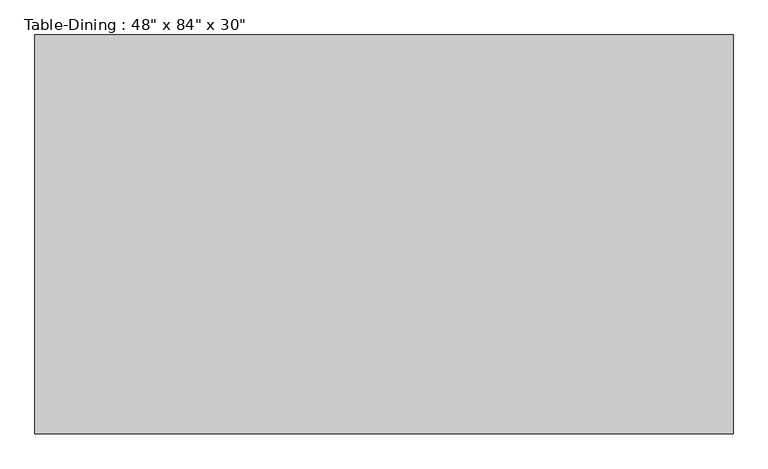
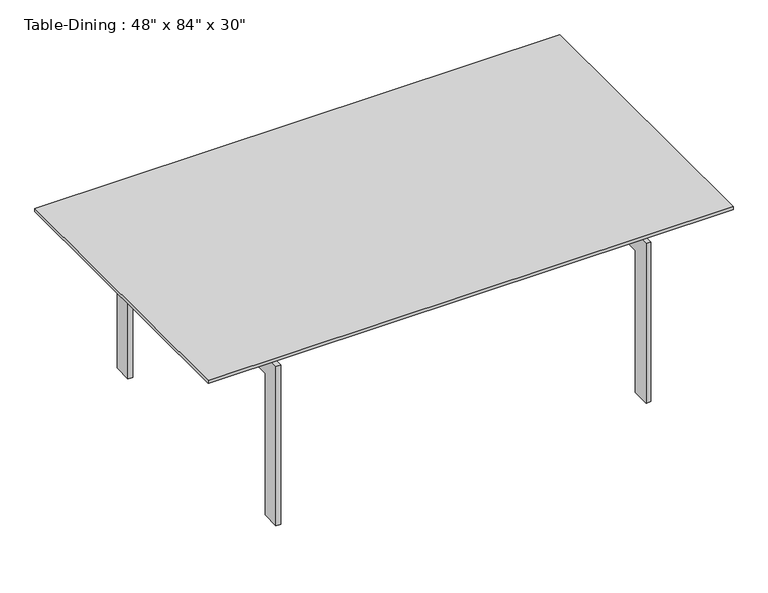
"""IFC4 building model written with IfcOpenShell, lengths in millimetres: furniture geometry."""

import ifcopenshell
import ifcopenshell.guid

model = None  # the IFC model being written
_history = None  # IfcOwnerHistory: only IFC2X3 demands one
_inside = {}  # id of a spatial element -> (the spatial element, [elements in it])
_under = {}  # id of a project, library or spatial element -> (it, [spatial elements below it])
_declared = {}  # id of a project -> (the project, [libraries it declares])
_typed = {}  # id of a type object -> (the type object, [elements of that type])
_made_of = {}  # id of a material, layer set ... -> (it, [elements and type objects made of it])


def new_model(schema):
    """Start an empty IFC model of exactly this schema.

    Asked for "IFC4X3", IfcOpenShell would pick the latest addendum, in which some entities
    have other attributes; the version numbers below select the first issue.
    IFC2X3 requires an IfcOwnerHistory on every rooted entity: one is made here for all.
    """
    global model, _history
    if schema == "IFC4X3":
        model = ifcopenshell.file(schema_version=(4, 3, 0, 0))
    else:
        model = ifcopenshell.file(schema=schema)
    _inside.clear()
    _under.clear()
    _declared.clear()
    _typed.clear()
    _made_of.clear()
    _history = None
    if model.schema == "IFC2X3":
        org = make("IfcOrganization", Name="unknown")
        user = make(
            "IfcPersonAndOrganization",
            ThePerson=make("IfcPerson", FamilyName="unknown"),
            TheOrganization=org,
        )
        app = make(
            "IfcApplication",
            ApplicationDeveloper=org,
            Version="unknown",
            ApplicationFullName="unknown",
            ApplicationIdentifier="unknown",
        )
        _history = make(
            "IfcOwnerHistory",
            OwningUser=user,
            OwningApplication=app,
            ChangeAction="ADDED",
            CreationDate=0,
        )
    return model


def make(cls, **values):
    """One entity of the class cls with the attributes given. An attribute that is None is left unset."""
    return model.create_entity(
        cls, **{name: value for name, value in values.items() if value is not None}
    )


def rooted(cls, **values):
    """An entity with a GlobalId (a new one), such as an element, a storey or a relation."""
    return make(cls, GlobalId=ifcopenshell.guid.new(), OwnerHistory=_history, **values)


def si_unit(unit_type, name, prefix=None):
    """IfcSIUnit, for example si_unit("LENGTHUNIT", "METRE", prefix="MILLI")."""
    return make("IfcSIUnit", UnitType=unit_type, Prefix=prefix, Name=name)


def assignment(units):
    """IfcUnitAssignment: the units of a project."""
    return None if units is None else make("IfcUnitAssignment", Units=units)


def point(xyz):
    """IfcCartesianPoint."""
    return None if xyz is None else make("IfcCartesianPoint", Coordinates=xyz)


def direction(xyz):
    """IfcDirection."""
    return None if xyz is None else make("IfcDirection", DirectionRatios=xyz)


def frame(location, z_axis=None, x_axis=None):
    """IfcAxis2Placement3D, a coordinate frame: its origin and axes. An axis left out is left unset."""
    return make(
        "IfcAxis2Placement3D",
        Location=point(location),
        Axis=direction(z_axis),
        RefDirection=direction(x_axis),
    )


def origin():
    """The frame at (0, 0, 0) with its axes left unset."""
    return frame((0.0, 0.0, 0.0))


def place(relative_to, where):
    """IfcLocalPlacement: puts the frame where relative to a parent placement (None: the world)."""
    return make(
        "IfcLocalPlacement", PlacementRelTo=relative_to, RelativePlacement=where
    )


def context(
    kind, dimensions, precision=None, world=None, true_north=None, identifier=None
):
    """IfcGeometricRepresentationContext, for example the 3D "Model" context."""
    return make(
        "IfcGeometricRepresentationContext",
        ContextIdentifier=identifier,
        ContextType=kind,
        CoordinateSpaceDimension=dimensions,
        Precision=precision,
        WorldCoordinateSystem=world,
        TrueNorth=true_north,
    )


def project(units=None, contexts=None):
    """IfcProject with its units and contexts."""
    return rooted(
        "IfcProject",
        Name="project",
        RepresentationContexts=contexts,
        UnitsInContext=assignment(units),
    )


def spatial(cls, under=None, at=None, **own):
    """A site, building, storey or space (cls), placed at a placement, below another one or the project."""
    s = rooted(cls, ObjectPlacement=at, **own)
    if under is not None:
        _under.setdefault(under.id(), (under, []))[1].append(s)
    return s


def polyline(points):
    """IfcPolyline through the points."""
    return make("IfcPolyline", Points=[point(p) for p in points])


def outline(outer, holes=None, kind="AREA"):
    """IfcArbitraryClosedProfileDef: a profile drawn as a closed curve; with holes, ...WithVoids."""
    if holes is None:
        return make("IfcArbitraryClosedProfileDef", ProfileType=kind, OuterCurve=outer)
    return make(
        "IfcArbitraryProfileDefWithVoids",
        ProfileType=kind,
        OuterCurve=outer,
        InnerCurves=holes,
    )


def extrude(swept, where, along, depth):
    """IfcExtrudedAreaSolid: the profile swept, set in the frame where, extruded along a direction by depth."""
    return make(
        "IfcExtrudedAreaSolid",
        SweptArea=swept,
        Position=where,
        ExtrudedDirection=direction(along),
        Depth=depth,
    )


def shape(context_of_items, identifier, shape_type, items):
    """IfcShapeRepresentation: the items that make up one representation, for example the "Body"."""
    return make(
        "IfcShapeRepresentation",
        ContextOfItems=context_of_items,
        RepresentationIdentifier=identifier,
        RepresentationType=shape_type,
        Items=items,
    )


def source(mapping_origin, context_of_items, identifier, shape_type, items):
    """IfcRepresentationMap: a shape defined once, which mapped items show again and again."""
    return make(
        "IfcRepresentationMap",
        MappingOrigin=mapping_origin,
        MappedRepresentation=shape(context_of_items, identifier, shape_type, items),
    )


def transform(
    local_origin,
    x_axis=None,
    y_axis=None,
    z_axis=None,
    scale=None,
    scale2=None,
    scale3=None,
    uniform=True,
):
    """IfcCartesianTransformationOperator3D, or its non-uniform kind. x_axis, y_axis, z_axis: its Axis1, 2, 3."""
    if uniform:
        return make(
            "IfcCartesianTransformationOperator3D",
            Axis1=direction(x_axis),
            Axis2=direction(y_axis),
            LocalOrigin=point(local_origin),
            Scale=scale,
            Axis3=direction(z_axis),
        )
    return make(
        "IfcCartesianTransformationOperator3DnonUniform",
        Axis1=direction(x_axis),
        Axis2=direction(y_axis),
        LocalOrigin=point(local_origin),
        Scale=scale,
        Axis3=direction(z_axis),
        Scale2=scale2,
        Scale3=scale3,
    )


def mapped(mapping_source, mapping_target):
    """IfcMappedItem: shows the shape of a source again, moved by a transform."""
    return make(
        "IfcMappedItem", MappingSource=mapping_source, MappingTarget=mapping_target
    )


def made_of(thing, what):
    """Note that an element or type object is made of a material, layer set ...; save() writes the relation."""
    if what is not None:
        _made_of.setdefault(what.id(), (what, []))[1].append(thing)
    return thing


def element(
    cls,
    number,
    at=None,
    inside=None,
    cuts=None,
    type_object=None,
    material=None,
    context=None,
    identifier="Body",
    shape_type=None,
    held_by="IfcProductDefinitionShape",
    body=None,
    shapes=None,
    **own,
):
    """One element of the class cls, such as IfcWall. Its Tag is "e" and its number.

    at: its placement. inside: the storey or other place that contains it. cuts: it is an
    opening in that element (IfcRelVoidsElement). A single representation is given by context,
    identifier, shape_type and body (its items); several are given by shapes. held_by: the class
    of the entity that holds the representations. save() writes the other relations.
    """
    e = rooted(cls, Tag="e%d" % number, ObjectPlacement=at, **own)
    if body is not None:
        shapes = [shape(context, identifier, shape_type, body)]
    if shapes is not None:
        e.Representation = make(held_by, Representations=shapes)
    if inside is not None:
        _inside.setdefault(inside.id(), (inside, []))[1].append(e)
    if cuts is not None:
        rooted(
            "IfcRelVoidsElement", RelatingBuildingElement=cuts, RelatedOpeningElement=e
        )
    if type_object is not None:
        _typed.setdefault(type_object.id(), (type_object, []))[1].append(e)
    return made_of(e, material)


def aggregate(whole, parts):
    """IfcRelAggregates: a whole, such as a stair, and the parts it consists of."""
    return rooted("IfcRelAggregates", RelatingObject=whole, RelatedObjects=parts)


def save(model, path):
    """Write the relations noted so far, then the file.

    IfcRelAggregates (storeys below a building ...), IfcRelContainedInSpatialStructure (elements
    in a storey), IfcRelDefinesByType, IfcRelAssociatesMaterial and IfcRelDeclares: one each for
    every whole, place, type object, material and project.
    """
    for whole, parts in _under.values():
        aggregate(whole, parts)
    for where, things in _inside.values():
        rooted(
            "IfcRelContainedInSpatialStructure",
            RelatedElements=things,
            RelatingStructure=where,
        )
    for kind, things in _typed.values():
        rooted("IfcRelDefinesByType", RelatedObjects=things, RelatingType=kind)
    for what, things in _made_of.values():
        rooted("IfcRelAssociatesMaterial", RelatedObjects=things, RelatingMaterial=what)
    for by, libraries in _declared.values():
        rooted("IfcRelDeclares", RelatingContext=by, RelatedDefinitions=libraries)
    model.write(path)


def furniture_c1a6d451(model_context):
    return source(origin(), model_context, "Body", "SweptSolid", [
        extrude(outline(polyline([(983.4657667, 297.7823857), (983.4657667, 272.3823857), (-946.9342333, 272.3823857), (-946.9342333, 297.7823857), (983.4657667, 297.7823857)])), frame((0.0, 0.0, 685.8), z_axis=(0.0, 0.0, 1.0), x_axis=(1.0, 0.0, 0.0)), (0.0, 0.0, 1.0), 63.5),
        extrude(outline(polyline([(983.4657667, -82.5889222), (983.4657667, -107.9889222), (-946.9342333, -107.9889222), (-946.9342333, -82.5889222), (983.4657667, -82.5889222)])), frame((0.0, 0.0, 685.8), z_axis=(0.0, 0.0, 1.0), x_axis=(1.0, 0.0, 0.0)), (0.0, 0.0, 1.0), 63.5),
        extrude(outline(polyline([(654.0110778, 0.0), (577.8110778, 0.0), (577.8110778, 609.6), (-387.3889222, 609.6), (-387.3889222, 0.0), (-463.5889222, 0.0), (-463.5889222, 685.8), (654.0110778, 685.8), (654.0110778, 0.0)])), frame((761.2157667, 0.0, 0.0), z_axis=(1.0, 0.0, 0.0), x_axis=(0.0, 1.0, 0.0)), (0.0, 0.0, 1.0), 19.05),
        extrude(outline(polyline([(654.0110778, 685.8), (654.0110778, 0.0), (577.8110778, 0.0), (577.8110778, 609.6), (-387.3889222, 609.6), (-387.3889222, 0.0), (-463.5889222, 0.0), (-463.5889222, 685.8), (654.0110778, 685.8)])), frame((-743.7342333, 0.0, 0.0), z_axis=(1.0, 0.0, 0.0), x_axis=(0.0, 1.0, 0.0)), (0.0, 0.0, 1.0), 19.05),
        extrude(outline(polyline([(1085.0657667, 704.8110778), (1085.0657667, -514.3889222), (-1048.5342333, -514.3889222), (-1048.5342333, 704.8110778), (1085.0657667, 704.8110778)])), frame((0.0, 0.0, 749.3), z_axis=(0.0, 0.0, 1.0), x_axis=(1.0, 0.0, 0.0)), (0.0, 0.0, 1.0), 12.7),
    ])


if __name__ == "__main__":
    model = new_model("IFC4")
    model_context = context("Model", 3, world=origin())
    ifc_project = project(units=[si_unit("LENGTHUNIT", "METRE", prefix="MILLI")], contexts=[model_context])
    site = spatial("IfcSite", under=ifc_project)
    building = spatial("IfcBuilding", under=site)
    placement = place(None, origin())
    furniture_shape = furniture_c1a6d451(model_context)
    element("IfcFurniture", 1, ObjectType="Table-Dining : 48\" x 84\" x 30\"", at=placement, inside=building, context=model_context, shape_type="MappedRepresentation", body=[
        mapped(furniture_shape, transform((0.0, 0.0, 0.0), x_axis=(1.0, 0.0, 0.0), y_axis=(0.0, 1.0, 0.0), z_axis=(0.0, 0.0, 1.0))),
    ])
    save(model, "model.ifc")

# Revit data of these elements
# Type "Table-Dining : 48\" x 84\" x 30\""
#   Assembly Code = "E2020200"
#   Height = 2' - 6"
#   Length = 7' - 0"
#   Width = 4' - 0"
#   Base Material = Metal - Chrome
#   Top Material = Wood - Birch
# Element 1 (IfcFurniture, "Table-Dining : 48\" x 84\" x 30\"")
#   Materials on its faces: "Metal - Chrome", "Wood - Birch"
# Materials
#   "Metal - Chrome": class "Metal", colour RGB 244 244 244, transparency 0, Comments = "Rendering appearance not upgraded Rendering appearance not upgraded ", Description = "Chrome"
#   "Wood - Birch": class "Wood", colour RGB 185 153 119, transparency 0, Comments = "Rendering appearance not upgraded Rendering appearance not upgraded "
